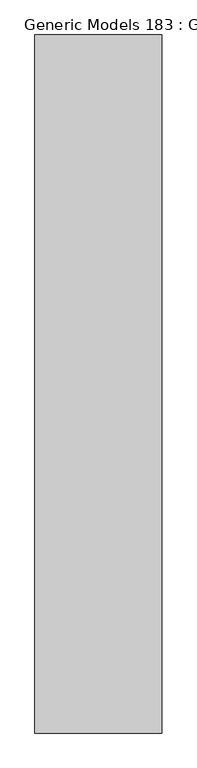
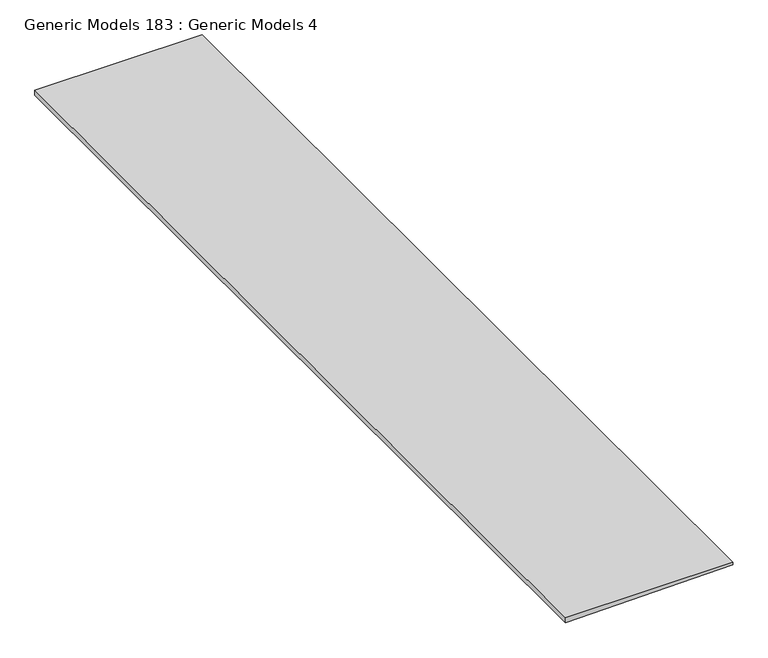
"""IFC4 building model written with IfcOpenShell, lengths in millimetres: proxy geometry, Generic Models 183 : Generic Models 4."""

from ifc_helpers import new_model, si_unit, frame, origin, place, context, project, spatial, polyline, outline, extrude, source, transform, mapped, element, save


def generic_models_183_generic_models_4_6fa96cc7(model_context):
    return source(origin(), model_context, "Body", "SweptSolid", [
        extrude(outline(polyline([(126748.56834, -6697.3784587), (126705.661417, -6697.3784587), (126729.51834, -5330.6162598), (126748.56834, -5330.6162598), (126748.56834, -6697.3784587)])), frame((0.0, -464.1230338, 0.0), z_axis=(0.0, 1.0, 0.0), x_axis=(0.0, 0.0, 1.0)), (0.0, 0.0, 1.0), 7518.4),
    ])


if __name__ == "__main__":
    model = new_model("IFC4")
    model_context = context("Model", 3, world=origin())
    ifc_project = project(units=[si_unit("LENGTHUNIT", "METRE", prefix="MILLI")], contexts=[model_context])
    site = spatial("IfcSite", under=ifc_project)
    building = spatial("IfcBuilding", under=site)
    placement = place(None, origin())
    generic_models_183_generic_models_4_shape = generic_models_183_generic_models_4_6fa96cc7(model_context)
    element("IfcBuildingElementProxy", 1, Name="Generic Models 183 : Generic Models 4", ObjectType="Generic Models 183 : Generic Models 4", at=placement, inside=building, context=model_context, shape_type="MappedRepresentation", body=[
        mapped(generic_models_183_generic_models_4_shape, transform((0.0, 0.0, 0.0), x_axis=(1.0, 0.0, 0.0), y_axis=(0.0, 1.0, 0.0), z_axis=(0.0, 0.0, 1.0))),
    ])
    save(model, "model.ifc")

# Revit data of these elements
# Element 1 (IfcBuildingElementProxy, "Generic Models 183 : Generic Models 4")
#   Materials on its faces: "_TAPERED TREATED 2X SLEEPERS (1% SLOPE)"
# Materials
#   "_TAPERED TREATED 2X SLEEPERS (1% SLOPE)": class "Generic", colour RGB 177 130 114, transparency 0, Cost = 0
